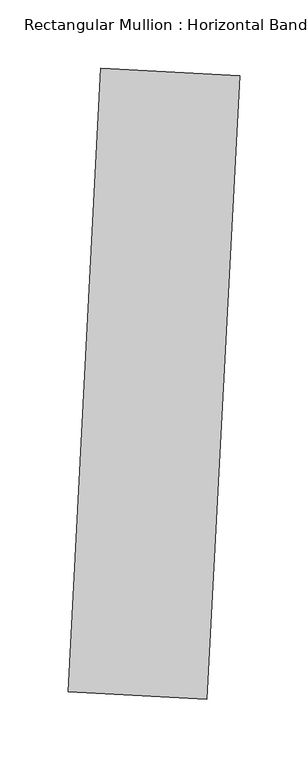
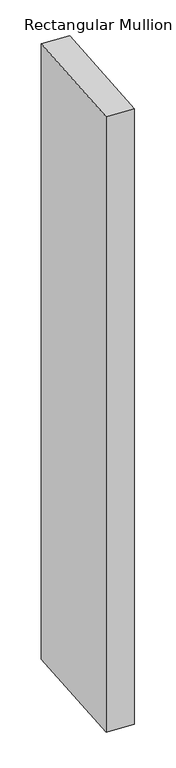
"""IFC4 building model written with IfcOpenShell, lengths in millimetres: member geometry, Rectangular Mullion : Horizontal Band."""

from ifc_helpers import new_model, si_unit, frame, origin, place, context, project, spatial, polyline, outline, extrude, source, transform, mapped, element, save


def rectangular_mullion_horizontal_band_5c9be954(model_context):
    return source(origin(), model_context, "Body", "SweptSolid", [
        extrude(outline(polyline([(62.69438, 301.8280451), (38.7663808, -154.7453782), (-62.69438, -149.4280451), (-38.7663808, 307.1453782), (62.69438, 301.8280451)])), frame((0.0, 0.0, -2412.0054926), z_axis=(0.0, 0.0, 1.0), x_axis=(1.0, 0.0, 0.0)), (0.0, 0.0, 1.0), 2412.0054926),
    ])


if __name__ == "__main__":
    model = new_model("IFC4")
    model_context = context("Model", 3, world=origin())
    ifc_project = project(units=[si_unit("LENGTHUNIT", "METRE", prefix="MILLI")], contexts=[model_context])
    site = spatial("IfcSite", under=ifc_project)
    building = spatial("IfcBuilding", under=site)
    placement = place(None, origin())
    rectangular_mullion_horizontal_band_shape = rectangular_mullion_horizontal_band_5c9be954(model_context)
    element("IfcMember", 1, ObjectType="Rectangular Mullion : Horizontal Band", at=placement, inside=building, context=model_context, shape_type="MappedRepresentation", body=[
        mapped(rectangular_mullion_horizontal_band_shape, transform((0.0, 0.0, 0.0), x_axis=(1.0, 0.0, 0.0), y_axis=(0.0, 1.0, 0.0), z_axis=(0.0, 0.0, 1.0))),
    ])
    save(model, "model.ifc")

# Revit data of these elements
# Type "Rectangular Mullion : Horizontal Band"
#   built-in parameter 1007351 = 0.25 (stored number, unit not read)
#   built-in parameter 1007304 = 1.5 (stored number, unit not read)
#   built-in parameter 1007301 = 0.166667 (stored number, unit not read)
#   built-in parameter 1007300 = 0.166667 (stored number, unit not read)
# Element 1 (IfcMember, "Rectangular Mullion : Horizontal Band")
#   Materials on its faces: "Aluminum"
# Materials
#   "Aluminum": class "Metal", colour RGB 247 247 247, transparency 0, Description = "Aluminum 6061", Cost = 0
